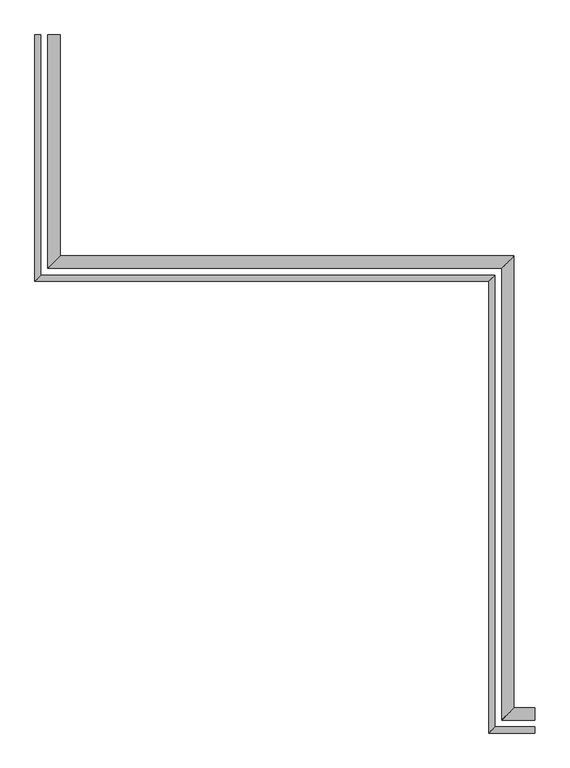
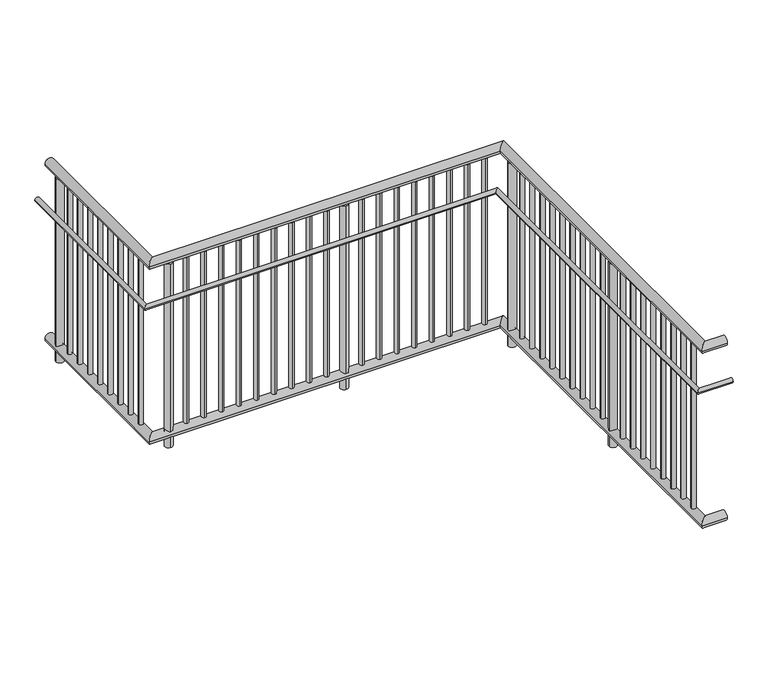
"""IFC4 building model written with IfcOpenShell, lengths in millimetres: railing geometry."""

from ifc_helpers import new_model, si_unit, point, frame, frame_2d, origin, place, context, project, spatial, circle_curve, ellipse_curve, trimmed, segment, composite_curve, outline, extrude, source, transform, mapped, element, save
from ifc_brep_helpers import plane_surface, cylinder_surface, advanced_brep


def railing_76a26c40(model_context):
    return source(origin(), model_context, "Body", "SolidModel", [
        advanced_brep(
        [(655.125551, -901.0965465, 4474.6), (604.325551, -901.0965465, 4474.6), (655.125551, -1825.6965465, 4474.6), (604.325551, -1876.4965465, 4474.6), (2555.125551, -1825.6965465, 4474.6), (2504.325551, -1876.4965465, 4474.6), (2555.125551, -3715.6965465, 4474.6), (2504.325551, -3766.4965465, 4474.6), (2643.025551, -3715.6965465, 4474.6), (2643.025551, -3766.4965465, 4474.6)],
        [
            (0, 1, circle_curve(frame((629.725551, -901.0965465, 4474.6), z_axis=(0.0, 1.0, 0.0), x_axis=(-1.0, 0.0, 0.0)), 25.4)),
            (1, 0, circle_curve(frame((629.725551, -901.0965465, 4474.6), z_axis=(0.0, 1.0, 0.0), x_axis=(-1.0, 0.0, 0.0)), 25.4)),
            (0, 2),
            (2, 3, ellipse_curve(frame((629.725551, -1851.0965465, 4474.6), z_axis=(-0.7071067811865475, 0.7071067811865475, 0.0), x_axis=(0.7071067811865474, 0.7071067811865476, 0.0)), 35.9210245, 25.4)),
            (3, 1),
            (3, 2, ellipse_curve(frame((629.725551, -1851.0965465, 4474.6), z_axis=(-0.7071067811865475, 0.7071067811865475, 0.0), x_axis=(0.7071067811865474, 0.7071067811865476, 0.0)), 35.9210245, 25.4)),
            (2, 4),
            (4, 5, ellipse_curve(frame((2529.725551, -1851.0965465, 4474.6), z_axis=(-0.7071067811865475, 0.7071067811865475, 0.0), x_axis=(-0.7071067811865476, -0.7071067811865474, 0.0)), 35.9210245, 25.4)),
            (5, 3),
            (5, 4, ellipse_curve(frame((2529.725551, -1851.0965465, 4474.6), z_axis=(-0.7071067811865475, 0.7071067811865475, 0.0), x_axis=(-0.7071067811865476, -0.7071067811865474, 0.0)), 35.9210245, 25.4)),
            (4, 6),
            (6, 7, ellipse_curve(frame((2529.725551, -3741.0965465, 4474.6), z_axis=(-0.7071067811865475, 0.7071067811865475, 0.0), x_axis=(0.7071067811865474, 0.7071067811865476, 0.0)), 35.9210245, 25.4)),
            (7, 5),
            (7, 6, ellipse_curve(frame((2529.725551, -3741.0965465, 4474.6), z_axis=(-0.7071067811865475, 0.7071067811865475, 0.0), x_axis=(0.7071067811865474, 0.7071067811865476, 0.0)), 35.9210245, 25.4)),
            (8, 9, circle_curve(frame((2643.025551, -3741.0965465, 4474.6), z_axis=(1.0, 0.0, 0.0), x_axis=(0.0, -1.0, 0.0)), 25.4)),
            (9, 8, circle_curve(frame((2643.025551, -3741.0965465, 4474.6), z_axis=(1.0, 0.0, 0.0), x_axis=(0.0, -1.0, 0.0)), 25.4)),
            (6, 8),
            (9, 7),
        ],
        [
            plane_surface(frame((629.725551, -901.0965465, 4500.0), z_axis=(0.0, 1.0, 0.0), x_axis=(0.0, 0.0, -1.0))),
            cylinder_surface(frame((629.725551, -901.0965465, 4474.6), z_axis=(0.0, 1.0, 0.0), x_axis=(-1.0, 0.0, 0.0)), 25.4),
            cylinder_surface(frame((629.725551, -1851.0965465, 4474.6), z_axis=(-1.0, 0.0, 0.0), x_axis=(0.0, -1.0, 0.0)), 25.4),
            cylinder_surface(frame((2529.725551, -1851.0965465, 4474.6), z_axis=(0.0, 1.0, 0.0), x_axis=(-1.0, 0.0, 0.0)), 25.4),
            plane_surface(frame((2643.025551, -3741.0965465, 4500.0), z_axis=(1.0, 0.0, 0.0), x_axis=(0.0, 1.0, 0.0))),
            cylinder_surface(frame((2529.725551, -3741.0965465, 4474.6), z_axis=(-1.0, 0.0, 0.0), x_axis=(0.0, -1.0, 0.0)), 25.4),
        ],
        [
            (0, [[1, 2]]),
            (1, [[-1, 3, 4, 5]]),
            (1, [[-2, -5, 6, -3]]),
            (2, [[-4, 7, 8, 9]]),
            (2, [[-6, -9, 10, -7]]),
            (3, [[-8, 11, 12, 13]]),
            (3, [[-10, -13, 14, -11]]),
            (4, [[15, 16]]),
            (5, [[-12, 17, -16, 18]]),
            (5, [[-14, -18, -15, -17]]),
        ],
    ),
        advanced_brep(
        [(575.425551, -901.0965465, 4287.3), (550.025551, -901.0965465, 4287.3), (575.425551, -1905.3965465, 4287.3), (550.025551, -1930.7965465, 4287.3), (2475.425551, -1905.3965465, 4287.3), (2450.025551, -1930.7965465, 4287.3), (2475.425551, -3795.3965465, 4287.3), (2450.025551, -3820.7965465, 4287.3), (2643.025551, -3795.3965465, 4287.3), (2643.025551, -3820.7965465, 4287.3)],
        [
            (0, 1, circle_curve(frame((562.725551, -901.0965465, 4287.3), z_axis=(0.0, 1.0, 0.0), x_axis=(-1.0, 0.0, 0.0)), 12.7)),
            (1, 0, circle_curve(frame((562.725551, -901.0965465, 4287.3), z_axis=(0.0, 1.0, 0.0), x_axis=(-1.0, 0.0, 0.0)), 12.7)),
            (0, 2),
            (2, 3, ellipse_curve(frame((562.725551, -1918.0965465, 4287.3), z_axis=(-0.7071067811865475, 0.7071067811865475, 0.0), x_axis=(0.7071067811865474, 0.7071067811865476, 0.0)), 17.9605122, 12.7)),
            (3, 1),
            (3, 2, ellipse_curve(frame((562.725551, -1918.0965465, 4287.3), z_axis=(-0.7071067811865475, 0.7071067811865475, 0.0), x_axis=(0.7071067811865474, 0.7071067811865476, 0.0)), 17.9605122, 12.7)),
            (2, 4),
            (4, 5, ellipse_curve(frame((2462.725551, -1918.0965465, 4287.3), z_axis=(-0.7071067811865475, 0.7071067811865475, 0.0), x_axis=(-0.7071067811865476, -0.7071067811865474, 0.0)), 17.9605122, 12.7)),
            (5, 3),
            (5, 4, ellipse_curve(frame((2462.725551, -1918.0965465, 4287.3), z_axis=(-0.7071067811865475, 0.7071067811865475, 0.0), x_axis=(-0.7071067811865476, -0.7071067811865474, 0.0)), 17.9605122, 12.7)),
            (4, 6),
            (6, 7, ellipse_curve(frame((2462.725551, -3808.0965465, 4287.3), z_axis=(-0.7071067811865475, 0.7071067811865475, 0.0), x_axis=(0.7071067811865474, 0.7071067811865476, 0.0)), 17.9605122, 12.7)),
            (7, 5),
            (7, 6, ellipse_curve(frame((2462.725551, -3808.0965465, 4287.3), z_axis=(-0.7071067811865475, 0.7071067811865475, 0.0), x_axis=(0.7071067811865474, 0.7071067811865476, 0.0)), 17.9605122, 12.7)),
            (8, 9, circle_curve(frame((2643.025551, -3808.0965465, 4287.3), z_axis=(1.0, 0.0, 0.0), x_axis=(0.0, -1.0, 0.0)), 12.7)),
            (9, 8, circle_curve(frame((2643.025551, -3808.0965465, 4287.3), z_axis=(1.0, 0.0, 0.0), x_axis=(0.0, -1.0, 0.0)), 12.7)),
            (6, 8),
            (9, 7),
        ],
        [
            plane_surface(frame((562.725551, -901.0965465, 4300.0), z_axis=(0.0, 1.0, 0.0), x_axis=(0.0, 0.0, -1.0))),
            cylinder_surface(frame((562.725551, -901.0965465, 4287.3), z_axis=(0.0, 1.0, 0.0), x_axis=(-1.0, 0.0, 0.0)), 12.7),
            cylinder_surface(frame((562.725551, -1918.0965465, 4287.3), z_axis=(-1.0, 0.0, 0.0), x_axis=(0.0, -1.0, 0.0)), 12.7),
            cylinder_surface(frame((2462.725551, -1918.0965465, 4287.3), z_axis=(0.0, 1.0, 0.0), x_axis=(-1.0, 0.0, 0.0)), 12.7),
            plane_surface(frame((2643.025551, -3808.0965465, 4300.0), z_axis=(1.0, 0.0, 0.0), x_axis=(0.0, 1.0, 0.0))),
            cylinder_surface(frame((2462.725551, -3808.0965465, 4287.3), z_axis=(-1.0, 0.0, 0.0), x_axis=(0.0, -1.0, 0.0)), 12.7),
        ],
        [
            (0, [[1, 2]]),
            (1, [[-1, 3, 4, 5]]),
            (1, [[-2, -5, 6, -3]]),
            (2, [[-4, 7, 8, 9]]),
            (2, [[-6, -9, 10, -7]]),
            (3, [[-8, 11, 12, 13]]),
            (3, [[-10, -13, 14, -11]]),
            (4, [[15, 16]]),
            (5, [[-12, 17, -16, 18]]),
            (5, [[-14, -18, -15, -17]]),
        ],
    ),
        advanced_brep(
        [(655.125551, -901.0965465, 3474.6), (604.325551, -901.0965465, 3474.6), (655.125551, -1825.6965465, 3474.6), (604.325551, -1876.4965465, 3474.6), (2555.125551, -1825.6965465, 3474.6), (2504.325551, -1876.4965465, 3474.6), (2555.125551, -3715.6965465, 3474.6), (2504.325551, -3766.4965465, 3474.6), (2643.025551, -3715.6965465, 3474.6), (2643.025551, -3766.4965465, 3474.6)],
        [
            (0, 1, circle_curve(frame((629.725551, -901.0965465, 3474.6), z_axis=(0.0, 1.0, 0.0), x_axis=(-1.0, 0.0, 0.0)), 25.4)),
            (1, 0, circle_curve(frame((629.725551, -901.0965465, 3474.6), z_axis=(0.0, 1.0, 0.0), x_axis=(-1.0, 0.0, 0.0)), 25.4)),
            (0, 2),
            (2, 3, ellipse_curve(frame((629.725551, -1851.0965465, 3474.6), z_axis=(-0.7071067811865475, 0.7071067811865475, 0.0), x_axis=(0.7071067811865474, 0.7071067811865476, 0.0)), 35.9210245, 25.4)),
            (3, 1),
            (3, 2, ellipse_curve(frame((629.725551, -1851.0965465, 3474.6), z_axis=(-0.7071067811865475, 0.7071067811865475, 0.0), x_axis=(0.7071067811865474, 0.7071067811865476, 0.0)), 35.9210245, 25.4)),
            (2, 4),
            (4, 5, ellipse_curve(frame((2529.725551, -1851.0965465, 3474.6), z_axis=(-0.7071067811865475, 0.7071067811865475, 0.0), x_axis=(-0.7071067811865476, -0.7071067811865474, 0.0)), 35.9210245, 25.4)),
            (5, 3),
            (5, 4, ellipse_curve(frame((2529.725551, -1851.0965465, 3474.6), z_axis=(-0.7071067811865475, 0.7071067811865475, 0.0), x_axis=(-0.7071067811865476, -0.7071067811865474, 0.0)), 35.9210245, 25.4)),
            (4, 6),
            (6, 7, ellipse_curve(frame((2529.725551, -3741.0965465, 3474.6), z_axis=(-0.7071067811865475, 0.7071067811865475, 0.0), x_axis=(0.7071067811865474, 0.7071067811865476, 0.0)), 35.9210245, 25.4)),
            (7, 5),
            (7, 6, ellipse_curve(frame((2529.725551, -3741.0965465, 3474.6), z_axis=(-0.7071067811865475, 0.7071067811865475, 0.0), x_axis=(0.7071067811865474, 0.7071067811865476, 0.0)), 35.9210245, 25.4)),
            (8, 9, circle_curve(frame((2643.025551, -3741.0965465, 3474.6), z_axis=(1.0, 0.0, 0.0), x_axis=(0.0, -1.0, 0.0)), 25.4)),
            (9, 8, circle_curve(frame((2643.025551, -3741.0965465, 3474.6), z_axis=(1.0, 0.0, 0.0), x_axis=(0.0, -1.0, 0.0)), 25.4)),
            (6, 8),
            (9, 7),
        ],
        [
            plane_surface(frame((629.725551, -901.0965465, 3500.0), z_axis=(0.0, 1.0, 0.0), x_axis=(0.0, 0.0, -1.0))),
            cylinder_surface(frame((629.725551, -901.0965465, 3474.6), z_axis=(0.0, 1.0, 0.0), x_axis=(-1.0, 0.0, 0.0)), 25.4),
            cylinder_surface(frame((629.725551, -1851.0965465, 3474.6), z_axis=(-1.0, 0.0, 0.0), x_axis=(0.0, -1.0, 0.0)), 25.4),
            cylinder_surface(frame((2529.725551, -1851.0965465, 3474.6), z_axis=(0.0, 1.0, 0.0), x_axis=(-1.0, 0.0, 0.0)), 25.4),
            plane_surface(frame((2643.025551, -3741.0965465, 3500.0), z_axis=(1.0, 0.0, 0.0), x_axis=(0.0, 1.0, 0.0))),
            cylinder_surface(frame((2529.725551, -3741.0965465, 3474.6), z_axis=(-1.0, 0.0, 0.0), x_axis=(0.0, -1.0, 0.0)), 25.4),
        ],
        [
            (0, [[1, 2]]),
            (1, [[-1, 3, 4, 5]]),
            (1, [[-2, -5, 6, -3]]),
            (2, [[-4, 7, 8, 9]]),
            (2, [[-6, -9, 10, -7]]),
            (3, [[-8, 11, 12, 13]]),
            (3, [[-10, -13, 14, -11]]),
            (4, [[15, 16]]),
            (5, [[-12, 17, -16, 18]]),
            (5, [[-14, -18, -15, -17]]),
        ],
    ),
        extrude(outline(composite_curve([segment(trimmed(circle_curve(frame_2d((2529.725551, -3646.5965465)), 12.5), [point((2542.225551, -3646.5965465))], [point((2517.225551, -3646.5965465))], False, "CARTESIAN"), True, "CONTINUOUS"), segment(trimmed(circle_curve(frame_2d((2529.725551, -3646.5965465)), 12.5), [point((2517.225551, -3646.5965465))], [point((2542.225551, -3646.5965465))], False, "CARTESIAN"), True, "CONTINUOUS")], self_intersect=False)), frame((0.0, 0.0, 3500.0), z_axis=(0.0, 0.0, 1.0), x_axis=(1.0, 0.0, 0.0)), (0.0, 0.0, 1.0), 949.2),
        extrude(outline(composite_curve([segment(trimmed(circle_curve(frame_2d((2529.725551, -3552.0965465)), 12.5), [point((2542.225551, -3552.0965465))], [point((2517.225551, -3552.0965465))], False, "CARTESIAN"), True, "CONTINUOUS"), segment(trimmed(circle_curve(frame_2d((2529.725551, -3552.0965465)), 12.5), [point((2517.225551, -3552.0965465))], [point((2542.225551, -3552.0965465))], False, "CARTESIAN"), True, "CONTINUOUS")], self_intersect=False)), frame((0.0, 0.0, 3500.0), z_axis=(0.0, 0.0, 1.0), x_axis=(1.0, 0.0, 0.0)), (0.0, 0.0, 1.0), 949.2),
        extrude(outline(composite_curve([segment(trimmed(circle_curve(frame_2d((2529.725551, -3457.5965465)), 12.5), [point((2542.225551, -3457.5965465))], [point((2517.225551, -3457.5965465))], False, "CARTESIAN"), True, "CONTINUOUS"), segment(trimmed(circle_curve(frame_2d((2529.725551, -3457.5965465)), 12.5), [point((2517.225551, -3457.5965465))], [point((2542.225551, -3457.5965465))], False, "CARTESIAN"), True, "CONTINUOUS")], self_intersect=False)), frame((0.0, 0.0, 3500.0), z_axis=(0.0, 0.0, 1.0), x_axis=(1.0, 0.0, 0.0)), (0.0, 0.0, 1.0), 949.2),
        extrude(outline(composite_curve([segment(trimmed(circle_curve(frame_2d((2529.725551, -3363.0965465)), 12.5), [point((2542.225551, -3363.0965465))], [point((2517.225551, -3363.0965465))], False, "CARTESIAN"), True, "CONTINUOUS"), segment(trimmed(circle_curve(frame_2d((2529.725551, -3363.0965465)), 12.5), [point((2517.225551, -3363.0965465))], [point((2542.225551, -3363.0965465))], False, "CARTESIAN"), True, "CONTINUOUS")], self_intersect=False)), frame((0.0, 0.0, 3500.0), z_axis=(0.0, 0.0, 1.0), x_axis=(1.0, 0.0, 0.0)), (0.0, 0.0, 1.0), 949.2),
        extrude(outline(composite_curve([segment(trimmed(circle_curve(frame_2d((2529.725551, -3268.5965465)), 12.5), [point((2542.225551, -3268.5965465))], [point((2517.225551, -3268.5965465))], False, "CARTESIAN"), True, "CONTINUOUS"), segment(trimmed(circle_curve(frame_2d((2529.725551, -3268.5965465)), 12.5), [point((2517.225551, -3268.5965465))], [point((2542.225551, -3268.5965465))], False, "CARTESIAN"), True, "CONTINUOUS")], self_intersect=False)), frame((0.0, 0.0, 3500.0), z_axis=(0.0, 0.0, 1.0), x_axis=(1.0, 0.0, 0.0)), (0.0, 0.0, 1.0), 949.2),
        extrude(outline(composite_curve([segment(trimmed(circle_curve(frame_2d((2529.725551, -3174.0965465)), 12.5), [point((2542.225551, -3174.0965465))], [point((2517.225551, -3174.0965465))], False, "CARTESIAN"), True, "CONTINUOUS"), segment(trimmed(circle_curve(frame_2d((2529.725551, -3174.0965465)), 12.5), [point((2517.225551, -3174.0965465))], [point((2542.225551, -3174.0965465))], False, "CARTESIAN"), True, "CONTINUOUS")], self_intersect=False)), frame((0.0, 0.0, 3500.0), z_axis=(0.0, 0.0, 1.0), x_axis=(1.0, 0.0, 0.0)), (0.0, 0.0, 1.0), 949.2),
        extrude(outline(composite_curve([segment(trimmed(circle_curve(frame_2d((2529.725551, -3079.5965465)), 12.5), [point((2542.225551, -3079.5965465))], [point((2517.225551, -3079.5965465))], False, "CARTESIAN"), True, "CONTINUOUS"), segment(trimmed(circle_curve(frame_2d((2529.725551, -3079.5965465)), 12.5), [point((2517.225551, -3079.5965465))], [point((2542.225551, -3079.5965465))], False, "CARTESIAN"), True, "CONTINUOUS")], self_intersect=False)), frame((0.0, 0.0, 3500.0), z_axis=(0.0, 0.0, 1.0), x_axis=(1.0, 0.0, 0.0)), (0.0, 0.0, 1.0), 949.2),
        extrude(outline(composite_curve([segment(trimmed(circle_curve(frame_2d((2529.725551, -2985.0965465)), 12.5), [point((2542.225551, -2985.0965465))], [point((2517.225551, -2985.0965465))], False, "CARTESIAN"), True, "CONTINUOUS"), segment(trimmed(circle_curve(frame_2d((2529.725551, -2985.0965465)), 12.5), [point((2517.225551, -2985.0965465))], [point((2542.225551, -2985.0965465))], False, "CARTESIAN"), True, "CONTINUOUS")], self_intersect=False)), frame((0.0, 0.0, 3500.0), z_axis=(0.0, 0.0, 1.0), x_axis=(1.0, 0.0, 0.0)), (0.0, 0.0, 1.0), 949.2),
        extrude(outline(composite_curve([segment(trimmed(circle_curve(frame_2d((2529.725551, -2890.5965465)), 21.0), [point((2550.725551, -2890.5965465))], [point((2508.725551, -2890.5965465))], False, "CARTESIAN"), True, "CONTINUOUS"), segment(trimmed(circle_curve(frame_2d((2529.725551, -2890.5965465)), 21.0), [point((2508.725551, -2890.5965465))], [point((2550.725551, -2890.5965465))], False, "CARTESIAN"), True, "CONTINUOUS")], self_intersect=False)), frame((0.0, 0.0, 3400.0), z_axis=(0.0, 0.0, 1.0), x_axis=(1.0, 0.0, 0.0)), (0.0, 0.0, 1.0), 1049.2),
        extrude(outline(composite_curve([segment(trimmed(circle_curve(frame_2d((2529.725551, -2796.0965465)), 12.5), [point((2542.225551, -2796.0965465))], [point((2517.225551, -2796.0965465))], False, "CARTESIAN"), True, "CONTINUOUS"), segment(trimmed(circle_curve(frame_2d((2529.725551, -2796.0965465)), 12.5), [point((2517.225551, -2796.0965465))], [point((2542.225551, -2796.0965465))], False, "CARTESIAN"), True, "CONTINUOUS")], self_intersect=False)), frame((0.0, 0.0, 3500.0), z_axis=(0.0, 0.0, 1.0), x_axis=(1.0, 0.0, 0.0)), (0.0, 0.0, 1.0), 949.2),
        extrude(outline(composite_curve([segment(trimmed(circle_curve(frame_2d((2529.725551, -2701.5965465)), 12.5), [point((2542.225551, -2701.5965465))], [point((2517.225551, -2701.5965465))], False, "CARTESIAN"), True, "CONTINUOUS"), segment(trimmed(circle_curve(frame_2d((2529.725551, -2701.5965465)), 12.5), [point((2517.225551, -2701.5965465))], [point((2542.225551, -2701.5965465))], False, "CARTESIAN"), True, "CONTINUOUS")], self_intersect=False)), frame((0.0, 0.0, 3500.0), z_axis=(0.0, 0.0, 1.0), x_axis=(1.0, 0.0, 0.0)), (0.0, 0.0, 1.0), 949.2),
        extrude(outline(composite_curve([segment(trimmed(circle_curve(frame_2d((2529.725551, -2607.0965465)), 12.5), [point((2542.225551, -2607.0965465))], [point((2517.225551, -2607.0965465))], False, "CARTESIAN"), True, "CONTINUOUS"), segment(trimmed(circle_curve(frame_2d((2529.725551, -2607.0965465)), 12.5), [point((2517.225551, -2607.0965465))], [point((2542.225551, -2607.0965465))], False, "CARTESIAN"), True, "CONTINUOUS")], self_intersect=False)), frame((0.0, 0.0, 3500.0), z_axis=(0.0, 0.0, 1.0), x_axis=(1.0, 0.0, 0.0)), (0.0, 0.0, 1.0), 949.2),
        extrude(outline(composite_curve([segment(trimmed(circle_curve(frame_2d((2529.725551, -2512.5965465)), 12.5), [point((2542.225551, -2512.5965465))], [point((2517.225551, -2512.5965465))], False, "CARTESIAN"), True, "CONTINUOUS"), segment(trimmed(circle_curve(frame_2d((2529.725551, -2512.5965465)), 12.5), [point((2517.225551, -2512.5965465))], [point((2542.225551, -2512.5965465))], False, "CARTESIAN"), True, "CONTINUOUS")], self_intersect=False)), frame((0.0, 0.0, 3500.0), z_axis=(0.0, 0.0, 1.0), x_axis=(1.0, 0.0, 0.0)), (0.0, 0.0, 1.0), 949.2),
        extrude(outline(composite_curve([segment(trimmed(circle_curve(frame_2d((2529.725551, -2418.0965465)), 12.5), [point((2542.225551, -2418.0965465))], [point((2517.225551, -2418.0965465))], False, "CARTESIAN"), True, "CONTINUOUS"), segment(trimmed(circle_curve(frame_2d((2529.725551, -2418.0965465)), 12.5), [point((2517.225551, -2418.0965465))], [point((2542.225551, -2418.0965465))], False, "CARTESIAN"), True, "CONTINUOUS")], self_intersect=False)), frame((0.0, 0.0, 3500.0), z_axis=(0.0, 0.0, 1.0), x_axis=(1.0, 0.0, 0.0)), (0.0, 0.0, 1.0), 949.2),
        extrude(outline(composite_curve([segment(trimmed(circle_curve(frame_2d((2529.725551, -2323.5965465)), 12.5), [point((2542.225551, -2323.5965465))], [point((2517.225551, -2323.5965465))], False, "CARTESIAN"), True, "CONTINUOUS"), segment(trimmed(circle_curve(frame_2d((2529.725551, -2323.5965465)), 12.5), [point((2517.225551, -2323.5965465))], [point((2542.225551, -2323.5965465))], False, "CARTESIAN"), True, "CONTINUOUS")], self_intersect=False)), frame((0.0, 0.0, 3500.0), z_axis=(0.0, 0.0, 1.0), x_axis=(1.0, 0.0, 0.0)), (0.0, 0.0, 1.0), 949.2),
        extrude(outline(composite_curve([segment(trimmed(circle_curve(frame_2d((2529.725551, -2229.0965465)), 12.5), [point((2542.225551, -2229.0965465))], [point((2517.225551, -2229.0965465))], False, "CARTESIAN"), True, "CONTINUOUS"), segment(trimmed(circle_curve(frame_2d((2529.725551, -2229.0965465)), 12.5), [point((2517.225551, -2229.0965465))], [point((2542.225551, -2229.0965465))], False, "CARTESIAN"), True, "CONTINUOUS")], self_intersect=False)), frame((0.0, 0.0, 3500.0), z_axis=(0.0, 0.0, 1.0), x_axis=(1.0, 0.0, 0.0)), (0.0, 0.0, 1.0), 949.2),
        extrude(outline(composite_curve([segment(trimmed(circle_curve(frame_2d((2529.725551, -2134.5965465)), 12.5), [point((2542.225551, -2134.5965465))], [point((2517.225551, -2134.5965465))], False, "CARTESIAN"), True, "CONTINUOUS"), segment(trimmed(circle_curve(frame_2d((2529.725551, -2134.5965465)), 12.5), [point((2517.225551, -2134.5965465))], [point((2542.225551, -2134.5965465))], False, "CARTESIAN"), True, "CONTINUOUS")], self_intersect=False)), frame((0.0, 0.0, 3500.0), z_axis=(0.0, 0.0, 1.0), x_axis=(1.0, 0.0, 0.0)), (0.0, 0.0, 1.0), 949.2),
        extrude(outline(composite_curve([segment(trimmed(circle_curve(frame_2d((2529.725551, -2040.0965465)), 12.5), [point((2542.225551, -2040.0965465))], [point((2517.225551, -2040.0965465))], False, "CARTESIAN"), True, "CONTINUOUS"), segment(trimmed(circle_curve(frame_2d((2529.725551, -2040.0965465)), 12.5), [point((2517.225551, -2040.0965465))], [point((2542.225551, -2040.0965465))], False, "CARTESIAN"), True, "CONTINUOUS")], self_intersect=False)), frame((0.0, 0.0, 3500.0), z_axis=(0.0, 0.0, 1.0), x_axis=(1.0, 0.0, 0.0)), (0.0, 0.0, 1.0), 949.2),
        extrude(outline(composite_curve([segment(trimmed(circle_curve(frame_2d((2529.725551, -1945.5965465)), 21.0), [point((2550.725551, -1945.5965465))], [point((2508.725551, -1945.5965465))], False, "CARTESIAN"), True, "CONTINUOUS"), segment(trimmed(circle_curve(frame_2d((2529.725551, -1945.5965465)), 21.0), [point((2508.725551, -1945.5965465))], [point((2550.725551, -1945.5965465))], False, "CARTESIAN"), True, "CONTINUOUS")], self_intersect=False)), frame((0.0, 0.0, 3400.0), z_axis=(0.0, 0.0, 1.0), x_axis=(1.0, 0.0, 0.0)), (0.0, 0.0, 1.0), 1049.2),
        extrude(outline(composite_curve([segment(trimmed(circle_curve(frame_2d((2434.725551, -1851.0965465)), 12.5), [point((2434.725551, -1838.5965465))], [point((2434.725551, -1863.5965465))], False, "CARTESIAN"), True, "CONTINUOUS"), segment(trimmed(circle_curve(frame_2d((2434.725551, -1851.0965465)), 12.5), [point((2434.725551, -1863.5965465))], [point((2434.725551, -1838.5965465))], False, "CARTESIAN"), True, "CONTINUOUS")], self_intersect=False)), frame((0.0, 0.0, 3500.0), z_axis=(0.0, 0.0, 1.0), x_axis=(1.0, 0.0, 0.0)), (0.0, 0.0, 1.0), 949.2),
        extrude(outline(composite_curve([segment(trimmed(circle_curve(frame_2d((2339.725551, -1851.0965465)), 12.5), [point((2339.725551, -1838.5965465))], [point((2339.725551, -1863.5965465))], False, "CARTESIAN"), True, "CONTINUOUS"), segment(trimmed(circle_curve(frame_2d((2339.725551, -1851.0965465)), 12.5), [point((2339.725551, -1863.5965465))], [point((2339.725551, -1838.5965465))], False, "CARTESIAN"), True, "CONTINUOUS")], self_intersect=False)), frame((0.0, 0.0, 3500.0), z_axis=(0.0, 0.0, 1.0), x_axis=(1.0, 0.0, 0.0)), (0.0, 0.0, 1.0), 949.2),
        extrude(outline(composite_curve([segment(trimmed(circle_curve(frame_2d((2244.725551, -1851.0965465)), 12.5), [point((2244.725551, -1838.5965465))], [point((2244.725551, -1863.5965465))], False, "CARTESIAN"), True, "CONTINUOUS"), segment(trimmed(circle_curve(frame_2d((2244.725551, -1851.0965465)), 12.5), [point((2244.725551, -1863.5965465))], [point((2244.725551, -1838.5965465))], False, "CARTESIAN"), True, "CONTINUOUS")], self_intersect=False)), frame((0.0, 0.0, 3500.0), z_axis=(0.0, 0.0, 1.0), x_axis=(1.0, 0.0, 0.0)), (0.0, 0.0, 1.0), 949.2),
        extrude(outline(composite_curve([segment(trimmed(circle_curve(frame_2d((2149.725551, -1851.0965465)), 12.5), [point((2149.725551, -1838.5965465))], [point((2149.725551, -1863.5965465))], False, "CARTESIAN"), True, "CONTINUOUS"), segment(trimmed(circle_curve(frame_2d((2149.725551, -1851.0965465)), 12.5), [point((2149.725551, -1863.5965465))], [point((2149.725551, -1838.5965465))], False, "CARTESIAN"), True, "CONTINUOUS")], self_intersect=False)), frame((0.0, 0.0, 3500.0), z_axis=(0.0, 0.0, 1.0), x_axis=(1.0, 0.0, 0.0)), (0.0, 0.0, 1.0), 949.2),
        extrude(outline(composite_curve([segment(trimmed(circle_curve(frame_2d((2054.725551, -1851.0965465)), 12.5), [point((2054.725551, -1838.5965465))], [point((2054.725551, -1863.5965465))], False, "CARTESIAN"), True, "CONTINUOUS"), segment(trimmed(circle_curve(frame_2d((2054.725551, -1851.0965465)), 12.5), [point((2054.725551, -1863.5965465))], [point((2054.725551, -1838.5965465))], False, "CARTESIAN"), True, "CONTINUOUS")], self_intersect=False)), frame((0.0, 0.0, 3500.0), z_axis=(0.0, 0.0, 1.0), x_axis=(1.0, 0.0, 0.0)), (0.0, 0.0, 1.0), 949.2),
        extrude(outline(composite_curve([segment(trimmed(circle_curve(frame_2d((1959.725551, -1851.0965465)), 12.5), [point((1959.725551, -1838.5965465))], [point((1959.725551, -1863.5965465))], False, "CARTESIAN"), True, "CONTINUOUS"), segment(trimmed(circle_curve(frame_2d((1959.725551, -1851.0965465)), 12.5), [point((1959.725551, -1863.5965465))], [point((1959.725551, -1838.5965465))], False, "CARTESIAN"), True, "CONTINUOUS")], self_intersect=False)), frame((0.0, 0.0, 3500.0), z_axis=(0.0, 0.0, 1.0), x_axis=(1.0, 0.0, 0.0)), (0.0, 0.0, 1.0), 949.2),
        extrude(outline(composite_curve([segment(trimmed(circle_curve(frame_2d((1864.725551, -1851.0965465)), 12.5), [point((1864.725551, -1838.5965465))], [point((1864.725551, -1863.5965465))], False, "CARTESIAN"), True, "CONTINUOUS"), segment(trimmed(circle_curve(frame_2d((1864.725551, -1851.0965465)), 12.5), [point((1864.725551, -1863.5965465))], [point((1864.725551, -1838.5965465))], False, "CARTESIAN"), True, "CONTINUOUS")], self_intersect=False)), frame((0.0, 0.0, 3500.0), z_axis=(0.0, 0.0, 1.0), x_axis=(1.0, 0.0, 0.0)), (0.0, 0.0, 1.0), 949.2),
        extrude(outline(composite_curve([segment(trimmed(circle_curve(frame_2d((1769.725551, -1851.0965465)), 12.5), [point((1769.725551, -1838.5965465))], [point((1769.725551, -1863.5965465))], False, "CARTESIAN"), True, "CONTINUOUS"), segment(trimmed(circle_curve(frame_2d((1769.725551, -1851.0965465)), 12.5), [point((1769.725551, -1863.5965465))], [point((1769.725551, -1838.5965465))], False, "CARTESIAN"), True, "CONTINUOUS")], self_intersect=False)), frame((0.0, 0.0, 3500.0), z_axis=(0.0, 0.0, 1.0), x_axis=(1.0, 0.0, 0.0)), (0.0, 0.0, 1.0), 949.2),
        extrude(outline(composite_curve([segment(trimmed(circle_curve(frame_2d((1674.725551, -1851.0965465)), 21.0), [point((1674.725551, -1830.0965465))], [point((1674.725551, -1872.0965465))], False, "CARTESIAN"), True, "CONTINUOUS"), segment(trimmed(circle_curve(frame_2d((1674.725551, -1851.0965465)), 21.0), [point((1674.725551, -1872.0965465))], [point((1674.725551, -1830.0965465))], False, "CARTESIAN"), True, "CONTINUOUS")], self_intersect=False)), frame((0.0, 0.0, 3400.0), z_axis=(0.0, 0.0, 1.0), x_axis=(1.0, 0.0, 0.0)), (0.0, 0.0, 1.0), 1049.2),
        extrude(outline(composite_curve([segment(trimmed(circle_curve(frame_2d((1579.725551, -1851.0965465)), 12.5), [point((1579.725551, -1838.5965465))], [point((1579.725551, -1863.5965465))], False, "CARTESIAN"), True, "CONTINUOUS"), segment(trimmed(circle_curve(frame_2d((1579.725551, -1851.0965465)), 12.5), [point((1579.725551, -1863.5965465))], [point((1579.725551, -1838.5965465))], False, "CARTESIAN"), True, "CONTINUOUS")], self_intersect=False)), frame((0.0, 0.0, 3500.0), z_axis=(0.0, 0.0, 1.0), x_axis=(1.0, 0.0, 0.0)), (0.0, 0.0, 1.0), 949.2),
        extrude(outline(composite_curve([segment(trimmed(circle_curve(frame_2d((1484.725551, -1851.0965465)), 12.5), [point((1484.725551, -1838.5965465))], [point((1484.725551, -1863.5965465))], False, "CARTESIAN"), True, "CONTINUOUS"), segment(trimmed(circle_curve(frame_2d((1484.725551, -1851.0965465)), 12.5), [point((1484.725551, -1863.5965465))], [point((1484.725551, -1838.5965465))], False, "CARTESIAN"), True, "CONTINUOUS")], self_intersect=False)), frame((0.0, 0.0, 3500.0), z_axis=(0.0, 0.0, 1.0), x_axis=(1.0, 0.0, 0.0)), (0.0, 0.0, 1.0), 949.2),
        extrude(outline(composite_curve([segment(trimmed(circle_curve(frame_2d((1389.725551, -1851.0965465)), 12.5), [point((1389.725551, -1838.5965465))], [point((1389.725551, -1863.5965465))], False, "CARTESIAN"), True, "CONTINUOUS"), segment(trimmed(circle_curve(frame_2d((1389.725551, -1851.0965465)), 12.5), [point((1389.725551, -1863.5965465))], [point((1389.725551, -1838.5965465))], False, "CARTESIAN"), True, "CONTINUOUS")], self_intersect=False)), frame((0.0, 0.0, 3500.0), z_axis=(0.0, 0.0, 1.0), x_axis=(1.0, 0.0, 0.0)), (0.0, 0.0, 1.0), 949.2),
        extrude(outline(composite_curve([segment(trimmed(circle_curve(frame_2d((1294.725551, -1851.0965465)), 12.5), [point((1294.725551, -1838.5965465))], [point((1294.725551, -1863.5965465))], False, "CARTESIAN"), True, "CONTINUOUS"), segment(trimmed(circle_curve(frame_2d((1294.725551, -1851.0965465)), 12.5), [point((1294.725551, -1863.5965465))], [point((1294.725551, -1838.5965465))], False, "CARTESIAN"), True, "CONTINUOUS")], self_intersect=False)), frame((0.0, 0.0, 3500.0), z_axis=(0.0, 0.0, 1.0), x_axis=(1.0, 0.0, 0.0)), (0.0, 0.0, 1.0), 949.2),
        extrude(outline(composite_curve([segment(trimmed(circle_curve(frame_2d((1199.725551, -1851.0965465)), 12.5), [point((1199.725551, -1838.5965465))], [point((1199.725551, -1863.5965465))], False, "CARTESIAN"), True, "CONTINUOUS"), segment(trimmed(circle_curve(frame_2d((1199.725551, -1851.0965465)), 12.5), [point((1199.725551, -1863.5965465))], [point((1199.725551, -1838.5965465))], False, "CARTESIAN"), True, "CONTINUOUS")], self_intersect=False)), frame((0.0, 0.0, 3500.0), z_axis=(0.0, 0.0, 1.0), x_axis=(1.0, 0.0, 0.0)), (0.0, 0.0, 1.0), 949.2),
        extrude(outline(composite_curve([segment(trimmed(circle_curve(frame_2d((1104.725551, -1851.0965465)), 12.5), [point((1104.725551, -1838.5965465))], [point((1104.725551, -1863.5965465))], False, "CARTESIAN"), True, "CONTINUOUS"), segment(trimmed(circle_curve(frame_2d((1104.725551, -1851.0965465)), 12.5), [point((1104.725551, -1863.5965465))], [point((1104.725551, -1838.5965465))], False, "CARTESIAN"), True, "CONTINUOUS")], self_intersect=False)), frame((0.0, 0.0, 3500.0), z_axis=(0.0, 0.0, 1.0), x_axis=(1.0, 0.0, 0.0)), (0.0, 0.0, 1.0), 949.2),
        extrude(outline(composite_curve([segment(trimmed(circle_curve(frame_2d((1009.725551, -1851.0965465)), 12.5), [point((1009.725551, -1838.5965465))], [point((1009.725551, -1863.5965465))], False, "CARTESIAN"), True, "CONTINUOUS"), segment(trimmed(circle_curve(frame_2d((1009.725551, -1851.0965465)), 12.5), [point((1009.725551, -1863.5965465))], [point((1009.725551, -1838.5965465))], False, "CARTESIAN"), True, "CONTINUOUS")], self_intersect=False)), frame((0.0, 0.0, 3500.0), z_axis=(0.0, 0.0, 1.0), x_axis=(1.0, 0.0, 0.0)), (0.0, 0.0, 1.0), 949.2),
        extrude(outline(composite_curve([segment(trimmed(circle_curve(frame_2d((914.725551, -1851.0965465)), 12.5), [point((914.725551, -1838.5965465))], [point((914.725551, -1863.5965465))], False, "CARTESIAN"), True, "CONTINUOUS"), segment(trimmed(circle_curve(frame_2d((914.725551, -1851.0965465)), 12.5), [point((914.725551, -1863.5965465))], [point((914.725551, -1838.5965465))], False, "CARTESIAN"), True, "CONTINUOUS")], self_intersect=False)), frame((0.0, 0.0, 3500.0), z_axis=(0.0, 0.0, 1.0), x_axis=(1.0, 0.0, 0.0)), (0.0, 0.0, 1.0), 949.2),
        extrude(outline(composite_curve([segment(trimmed(circle_curve(frame_2d((819.725551, -1851.0965465)), 12.5), [point((819.725551, -1838.5965465))], [point((819.725551, -1863.5965465))], False, "CARTESIAN"), True, "CONTINUOUS"), segment(trimmed(circle_curve(frame_2d((819.725551, -1851.0965465)), 12.5), [point((819.725551, -1863.5965465))], [point((819.725551, -1838.5965465))], False, "CARTESIAN"), True, "CONTINUOUS")], self_intersect=False)), frame((0.0, 0.0, 3500.0), z_axis=(0.0, 0.0, 1.0), x_axis=(1.0, 0.0, 0.0)), (0.0, 0.0, 1.0), 949.2),
        extrude(outline(composite_curve([segment(trimmed(circle_curve(frame_2d((724.725551, -1851.0965465)), 21.0), [point((724.725551, -1830.0965465))], [point((724.725551, -1872.0965465))], False, "CARTESIAN"), True, "CONTINUOUS"), segment(trimmed(circle_curve(frame_2d((724.725551, -1851.0965465)), 21.0), [point((724.725551, -1872.0965465))], [point((724.725551, -1830.0965465))], False, "CARTESIAN"), True, "CONTINUOUS")], self_intersect=False)), frame((0.0, 0.0, 3400.0), z_axis=(0.0, 0.0, 1.0), x_axis=(1.0, 0.0, 0.0)), (0.0, 0.0, 1.0), 1049.2),
        extrude(outline(composite_curve([segment(trimmed(circle_curve(frame_2d((629.725551, -1756.0965465)), 12.5), [point((642.225551, -1756.0965465))], [point((617.225551, -1756.0965465))], False, "CARTESIAN"), True, "CONTINUOUS"), segment(trimmed(circle_curve(frame_2d((629.725551, -1756.0965465)), 12.5), [point((617.225551, -1756.0965465))], [point((642.225551, -1756.0965465))], False, "CARTESIAN"), True, "CONTINUOUS")], self_intersect=False)), frame((0.0, 0.0, 3500.0), z_axis=(0.0, 0.0, 1.0), x_axis=(1.0, 0.0, 0.0)), (0.0, 0.0, 1.0), 949.2),
        extrude(outline(composite_curve([segment(trimmed(circle_curve(frame_2d((629.725551, -1661.0965465)), 12.5), [point((642.225551, -1661.0965465))], [point((617.225551, -1661.0965465))], False, "CARTESIAN"), True, "CONTINUOUS"), segment(trimmed(circle_curve(frame_2d((629.725551, -1661.0965465)), 12.5), [point((617.225551, -1661.0965465))], [point((642.225551, -1661.0965465))], False, "CARTESIAN"), True, "CONTINUOUS")], self_intersect=False)), frame((0.0, 0.0, 3500.0), z_axis=(0.0, 0.0, 1.0), x_axis=(1.0, 0.0, 0.0)), (0.0, 0.0, 1.0), 949.2),
        extrude(outline(composite_curve([segment(trimmed(circle_curve(frame_2d((629.725551, -1566.0965465)), 12.5), [point((642.225551, -1566.0965465))], [point((617.225551, -1566.0965465))], False, "CARTESIAN"), True, "CONTINUOUS"), segment(trimmed(circle_curve(frame_2d((629.725551, -1566.0965465)), 12.5), [point((617.225551, -1566.0965465))], [point((642.225551, -1566.0965465))], False, "CARTESIAN"), True, "CONTINUOUS")], self_intersect=False)), frame((0.0, 0.0, 3500.0), z_axis=(0.0, 0.0, 1.0), x_axis=(1.0, 0.0, 0.0)), (0.0, 0.0, 1.0), 949.2),
        extrude(outline(composite_curve([segment(trimmed(circle_curve(frame_2d((629.725551, -1471.0965465)), 12.5), [point((642.225551, -1471.0965465))], [point((617.225551, -1471.0965465))], False, "CARTESIAN"), True, "CONTINUOUS"), segment(trimmed(circle_curve(frame_2d((629.725551, -1471.0965465)), 12.5), [point((617.225551, -1471.0965465))], [point((642.225551, -1471.0965465))], False, "CARTESIAN"), True, "CONTINUOUS")], self_intersect=False)), frame((0.0, 0.0, 3500.0), z_axis=(0.0, 0.0, 1.0), x_axis=(1.0, 0.0, 0.0)), (0.0, 0.0, 1.0), 949.2),
        extrude(outline(composite_curve([segment(trimmed(circle_curve(frame_2d((629.725551, -1376.0965465)), 12.5), [point((642.225551, -1376.0965465))], [point((617.225551, -1376.0965465))], False, "CARTESIAN"), True, "CONTINUOUS"), segment(trimmed(circle_curve(frame_2d((629.725551, -1376.0965465)), 12.5), [point((617.225551, -1376.0965465))], [point((642.225551, -1376.0965465))], False, "CARTESIAN"), True, "CONTINUOUS")], self_intersect=False)), frame((0.0, 0.0, 3500.0), z_axis=(0.0, 0.0, 1.0), x_axis=(1.0, 0.0, 0.0)), (0.0, 0.0, 1.0), 949.2),
        extrude(outline(composite_curve([segment(trimmed(circle_curve(frame_2d((629.725551, -1281.0965465)), 12.5), [point((642.225551, -1281.0965465))], [point((617.225551, -1281.0965465))], False, "CARTESIAN"), True, "CONTINUOUS"), segment(trimmed(circle_curve(frame_2d((629.725551, -1281.0965465)), 12.5), [point((617.225551, -1281.0965465))], [point((642.225551, -1281.0965465))], False, "CARTESIAN"), True, "CONTINUOUS")], self_intersect=False)), frame((0.0, 0.0, 3500.0), z_axis=(0.0, 0.0, 1.0), x_axis=(1.0, 0.0, 0.0)), (0.0, 0.0, 1.0), 949.2),
        extrude(outline(composite_curve([segment(trimmed(circle_curve(frame_2d((629.725551, -1186.0965465)), 12.5), [point((642.225551, -1186.0965465))], [point((617.225551, -1186.0965465))], False, "CARTESIAN"), True, "CONTINUOUS"), segment(trimmed(circle_curve(frame_2d((629.725551, -1186.0965465)), 12.5), [point((617.225551, -1186.0965465))], [point((642.225551, -1186.0965465))], False, "CARTESIAN"), True, "CONTINUOUS")], self_intersect=False)), frame((0.0, 0.0, 3500.0), z_axis=(0.0, 0.0, 1.0), x_axis=(1.0, 0.0, 0.0)), (0.0, 0.0, 1.0), 949.2),
        extrude(outline(composite_curve([segment(trimmed(circle_curve(frame_2d((629.725551, -1091.0965465)), 12.5), [point((642.225551, -1091.0965465))], [point((617.225551, -1091.0965465))], False, "CARTESIAN"), True, "CONTINUOUS"), segment(trimmed(circle_curve(frame_2d((629.725551, -1091.0965465)), 12.5), [point((617.225551, -1091.0965465))], [point((642.225551, -1091.0965465))], False, "CARTESIAN"), True, "CONTINUOUS")], self_intersect=False)), frame((0.0, 0.0, 3500.0), z_axis=(0.0, 0.0, 1.0), x_axis=(1.0, 0.0, 0.0)), (0.0, 0.0, 1.0), 949.2),
        extrude(outline(composite_curve([segment(trimmed(circle_curve(frame_2d((629.725551, -996.0965465)), 21.0), [point((650.725551, -996.0965465))], [point((608.725551, -996.0965465))], False, "CARTESIAN"), True, "CONTINUOUS"), segment(trimmed(circle_curve(frame_2d((629.725551, -996.0965465)), 21.0), [point((608.725551, -996.0965465))], [point((650.725551, -996.0965465))], False, "CARTESIAN"), True, "CONTINUOUS")], self_intersect=False)), frame((0.0, 0.0, 3400.0), z_axis=(0.0, 0.0, 1.0), x_axis=(1.0, 0.0, 0.0)), (0.0, 0.0, 1.0), 1049.2),
    ])


if __name__ == "__main__":
    model = new_model("IFC4")
    model_context = context("Model", 3, world=origin())
    ifc_project = project(units=[si_unit("LENGTHUNIT", "METRE", prefix="MILLI")], contexts=[model_context])
    site = spatial("IfcSite", under=ifc_project)
    building = spatial("IfcBuilding", under=site)
    placement = place(None, origin())
    railing_shape = railing_76a26c40(model_context)
    element("IfcRailing", 1, at=placement, inside=building, context=model_context, shape_type="MappedRepresentation", body=[
        mapped(railing_shape, transform((0.0, 0.0, 0.0), x_axis=(1.0, 0.0, 0.0), y_axis=(0.0, 1.0, 0.0), z_axis=(0.0, 0.0, 1.0))),
    ])
    save(model, "model.ifc")

# Revit data of these elements
# Element 1 (IfcRailing)
#   Materials on its faces: "Ferro - Pintura Esmalte"
# Materials
#   "Ferro - Pintura Esmalte": class "Pintura", colour RGB 255 255 255, transparency 0, Cost = 0
